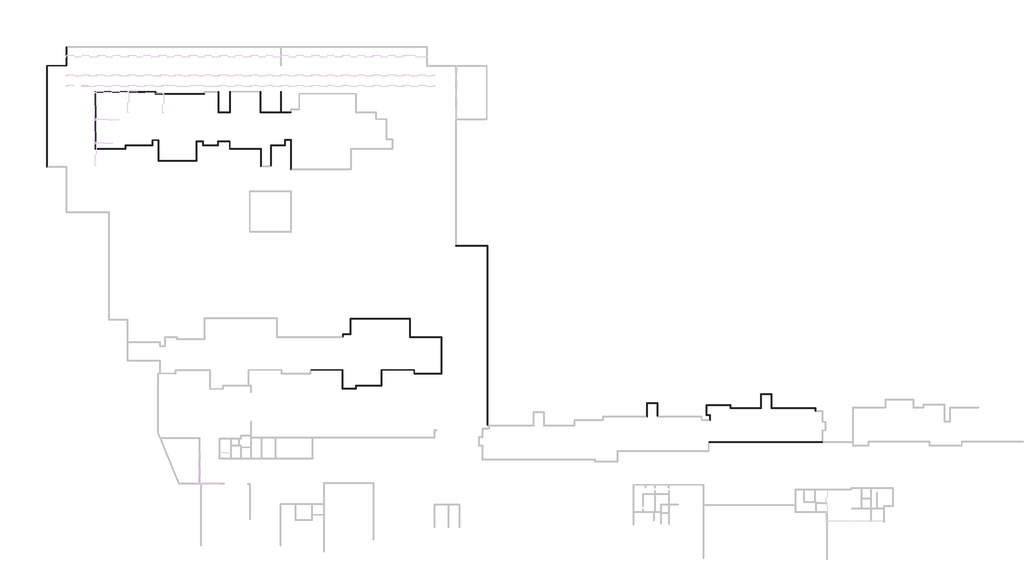
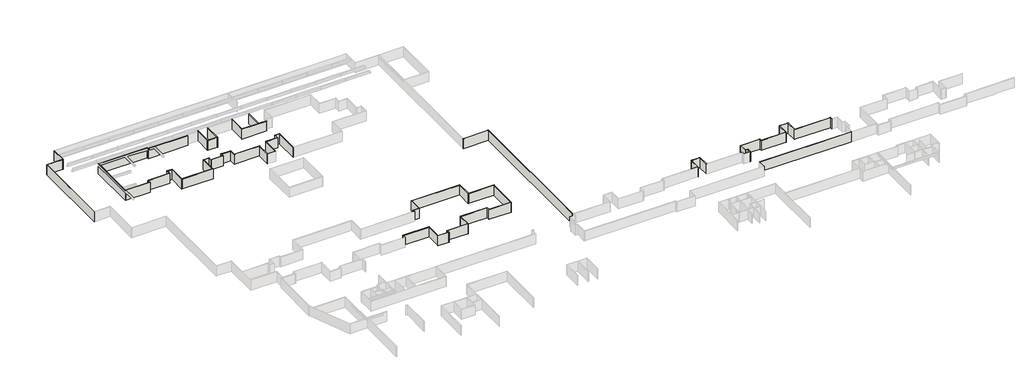
# One storey, part 5 of 8: 67 walls.
"""IFC4 building model written with IfcOpenShell, lengths in millimetres."""

from ifc_helpers import new_model, si_unit, origin, origin_with_axes, place, context, project, spatial, polyline, outline, extrude, faceted_brep, element, save

model = new_model("IFC4")

# Units and contexts
model_context = context("Model", 3, world=origin())
ifc_project = project(units=[si_unit("LENGTHUNIT", "METRE", prefix="MILLI")], contexts=[model_context])

# Site, building, storey
site = spatial("IfcSite", under=ifc_project)
building = spatial("IfcBuilding", under=site)
storey = spatial("IfcBuildingStorey", under=building, Name="户型图", Elevation=0.0)

# Walls
placement = place(None, origin())
element("IfcWall", 1, ObjectType="所有墙体", at=placement, inside=storey, context=model_context, shape_type="Brep", body=[
    faceted_brep([(57050.338145, 153057.0451916, 0.0), (57050.338145, 126907.0451941, 0.0), (57050.338145, 126907.0451941, 3300.0), (57050.338145, 153057.0451916, 3300.0), (57170.338145, 153057.0451916, 0.0), (57170.338145, 153057.0451916, 3300.0), (57170.338145, 127027.0451941, 3300.0), (57170.338145, 126907.0451941, 3300.0), (57170.338145, 126907.0451941, 0.0), (57170.338145, 127027.0451941, 0.0)], [[[0, 1, 2, 3]], [[4, 5, 6, 7, 8, 9]], [[1, 0, 4, 9, 8]], [[3, 2, 7, 6, 5]], [[2, 1, 8, 7]], [[0, 3, 5, 4]]]),
])
element("IfcWall", 2, ObjectType="所有墙体", at=placement, inside=storey, context=model_context, shape_type="Brep", body=[
    faceted_brep([(255784.4931741, 63876.5127734, 0.0), (255784.4931741, 64676.5110317, 0.0), (255784.4931741, 64676.5110317, 3300.0), (255784.4931741, 63876.5127734, 3300.0), (255664.4931741, 63876.5127734, 0.0), (255664.4931741, 63876.5127734, 3300.0), (255664.4931741, 64556.5110317, 3300.0), (255664.4931741, 64676.5110317, 3300.0), (255664.4931741, 64676.5110317, 0.0), (255664.4931741, 64556.5110317, 0.0)], [[[0, 1, 2, 3]], [[4, 5, 6, 7, 8, 9]], [[1, 0, 4, 9, 8]], [[3, 2, 7, 6, 5]], [[0, 3, 5, 4]], [[2, 1, 8, 7]]]),
])
element("IfcWall", 3, ObjectType="所有墙体", at=placement, inside=storey, context=model_context, shape_type="Brep", body=[
    faceted_brep([(255664.4931741, 64676.5110317, 0.0), (244359.4928017, 64676.5110317, 0.0), (244239.4928017, 64676.5110317, 0.0), (244239.4928017, 64676.5110317, 3300.0), (244359.4928017, 64676.5110317, 3300.0), (255664.4931741, 64676.5110317, 3300.0), (255664.4931741, 64556.5110317, 0.0), (255664.4931741, 64556.5110317, 3300.0), (244239.4928017, 64556.5110317, 3300.0), (244239.4928017, 64556.5110317, 0.0)], [[[0, 1, 2, 3, 4, 5]], [[6, 7, 8, 9]], [[2, 1, 0, 6, 9]], [[5, 4, 3, 8, 7]], [[0, 5, 7, 6]], [[3, 2, 9, 8]]]),
])
element("IfcWall", 4, ObjectType="所有墙体", at=placement, inside=storey, context=model_context, shape_type="Brep", body=[
    faceted_brep([(244359.4928017, 64676.5110317, 0.0), (244359.4928017, 68251.5115193, 0.0), (244359.4928017, 68251.5115193, 3300.0), (244359.4928017, 64676.5110317, 3300.0), (244239.4928017, 64676.5110317, 0.0), (244239.4928017, 64676.5110317, 3300.0), (244239.4928017, 68131.5115193, 3300.0), (244239.4928017, 68251.5115193, 3300.0), (244239.4928017, 68251.5115193, 0.0), (244239.4928017, 68131.5115193, 0.0)], [[[0, 1, 2, 3]], [[4, 5, 6, 7, 8, 9]], [[1, 0, 4, 9, 8]], [[3, 2, 7, 6, 5]], [[0, 3, 5, 4]], [[2, 1, 8, 7]]]),
])
element("IfcWall", 5, ObjectType="所有墙体", at=placement, inside=storey, context=model_context, shape_type="Brep", body=[
    faceted_brep([(244239.4928017, 68251.5115193, 0.0), (241539.4892961, 68251.5115193, 0.0), (241539.4892961, 68251.5115193, 3300.0), (244239.4928017, 68251.5115193, 3300.0), (244239.4928017, 68131.5115193, 0.0), (244239.4928017, 68131.5115193, 3300.0), (241659.4892961, 68131.5115193, 3300.0), (241539.4892961, 68131.5115193, 3300.0), (241539.4892961, 68131.5115193, 0.0), (241659.4892961, 68131.5115193, 0.0)], [[[0, 1, 2, 3]], [[4, 5, 6, 7, 8, 9]], [[1, 0, 4, 9, 8]], [[3, 2, 7, 6, 5]], [[0, 3, 5, 4]], [[2, 1, 8, 7]]]),
])
element("IfcWall", 6, ObjectType="所有墙体", at=placement, inside=storey, context=model_context, shape_type="Brep", body=[
    faceted_brep([(241539.4892961, 68131.5115193, 0.0), (241539.4892961, 64676.5110317, 0.0), (241539.4892961, 64556.5110317, 0.0), (241539.4892961, 64556.5110317, 3300.0), (241539.4892961, 64676.5110317, 3300.0), (241539.4892961, 68131.5115193, 3300.0), (241659.4892961, 68131.5115193, 0.0), (241659.4892961, 68131.5115193, 3300.0), (241659.4892961, 64556.5110317, 3300.0), (241659.4892961, 64556.5110317, 0.0)], [[[0, 1, 2, 3, 4, 5]], [[6, 7, 8, 9]], [[2, 1, 0, 6, 9]], [[5, 4, 3, 8, 7]], [[0, 5, 7, 6]], [[3, 2, 9, 8]]]),
])
element("IfcWall", 7, ObjectType="所有墙体", at=placement, inside=storey, context=model_context, shape_type="Brep", body=[
    faceted_brep([(241539.4892961, 64676.5110317, 0.0), (233784.2041334, 64676.5110317, 0.0), (233664.2041334, 64676.5110317, 0.0), (233664.2041334, 64676.5110317, 3300.0), (233784.2041334, 64676.5110317, 3300.0), (241539.4892961, 64676.5110317, 3300.0), (241539.4892961, 64556.5110317, 0.0), (241539.4892961, 64556.5110317, 3300.0), (233664.2041334, 64556.5110317, 3300.0), (233664.2041334, 64556.5110317, 0.0)], [[[0, 1, 2, 3, 4, 5]], [[6, 7, 8, 9]], [[2, 1, 0, 6, 9]], [[5, 4, 3, 8, 7]], [[0, 5, 7, 6]], [[3, 2, 9, 8]]]),
])
element("IfcWall", 8, ObjectType="所有墙体", at=placement, inside=storey, context=model_context, shape_type="Brep", body=[
    faceted_brep([(233784.2041334, 64676.5110317, 0.0), (233784.2041334, 65376.5510572, 0.0), (233784.2041334, 65376.5510572, 3300.0), (233784.2041334, 64676.5110317, 3300.0), (233664.2041334, 64676.5110317, 0.0), (233664.2041334, 64676.5110317, 3300.0), (233664.2041334, 65256.5510572, 3300.0), (233664.2041334, 65376.5510572, 3300.0), (233664.2041334, 65376.5510572, 0.0), (233664.2041334, 65256.5510572, 0.0)], [[[0, 1, 2, 3]], [[4, 5, 6, 7, 8, 9]], [[1, 0, 4, 9, 8]], [[3, 2, 7, 6, 5]], [[0, 3, 5, 4]], [[2, 1, 8, 7]]]),
])
element("IfcWall", 9, ObjectType="所有墙体", at=placement, inside=storey, context=model_context, shape_type="Brep", body=[
    faceted_brep([(233664.2041334, 65376.5510572, 0.0), (227494.4759798, 65376.5510572, 0.0), (227494.4759798, 65376.5510572, 3300.0), (233664.2041334, 65376.5510572, 3300.0), (233664.2041334, 65256.5510572, 0.0), (233664.2041334, 65256.5510572, 3300.0), (227614.4759798, 65256.5510572, 3300.0), (227494.4759798, 65256.5510572, 3300.0), (227494.4759798, 65256.5510572, 0.0), (227614.4759798, 65256.5510572, 0.0)], [[[0, 1, 2, 3]], [[4, 5, 6, 7, 8, 9]], [[1, 0, 4, 9, 8]], [[3, 2, 7, 6, 5]], [[0, 3, 5, 4]], [[2, 1, 8, 7]]]),
])
element("IfcWall", 10, ObjectType="所有墙体", at=placement, inside=storey, context=model_context, shape_type="Brep", body=[
    faceted_brep([(227494.4759798, 65256.5510572, 0.0), (227494.4759798, 62756.5107166, 0.0), (227494.4759798, 62756.5107166, 3300.0), (227494.4759798, 65256.5510572, 3300.0), (227614.4759798, 65256.5510572, 0.0), (227614.4759798, 65256.5510572, 3300.0), (227614.4759798, 62876.5107166, 3300.0), (227614.4759798, 62756.5107166, 3300.0), (227614.4759798, 62756.5107166, 0.0), (227614.4759798, 62876.5107166, 0.0)], [[[0, 1, 2, 3]], [[4, 5, 6, 7, 8, 9]], [[1, 0, 4, 9, 8]], [[3, 2, 7, 6, 5]], [[0, 3, 5, 4]], [[2, 1, 8, 7]]]),
])
element("IfcWall", 11, ObjectType="所有墙体", at=placement, inside=storey, context=model_context, shape_type="Brep", body=[
    faceted_brep([(227614.4759798, 62756.5107166, 0.0), (228364.4881621, 62756.5107166, 0.0), (228484.4881621, 62756.5107166, 0.0), (228484.4881621, 62756.5107166, 3300.0), (228364.4881621, 62756.5107166, 3300.0), (227614.4759798, 62756.5107166, 3300.0), (227614.4759798, 62876.5107166, 0.0), (227614.4759798, 62876.5107166, 3300.0), (228484.4881621, 62876.5107166, 3300.0), (228484.4881621, 62876.5107166, 0.0)], [[[0, 1, 2, 3, 4, 5]], [[6, 7, 8, 9]], [[2, 1, 0, 6, 9]], [[5, 4, 3, 8, 7]], [[0, 5, 7, 6]], [[3, 2, 9, 8]]]),
])
element("IfcWall", 12, ObjectType="所有墙体", at=placement, inside=storey, context=model_context, shape_type="Brep", body=[
    faceted_brep([(228364.4881621, 62756.5107166, 0.0), (228364.4881621, 61576.5107166, 0.0), (228364.4881621, 61456.5107166, 0.0), (228364.4881621, 61456.5107166, 3300.0), (228364.4881621, 61576.5107166, 3300.0), (228364.4881621, 62756.5107166, 3300.0), (228484.4881621, 62756.5107166, 0.0), (228484.4881621, 62756.5107166, 3300.0), (228484.4881621, 61456.5107166, 3300.0), (228484.4881621, 61456.5107166, 0.0)], [[[0, 1, 2, 3, 4, 5]], [[6, 7, 8, 9]], [[2, 1, 0, 6, 9]], [[5, 4, 3, 8, 7]], [[0, 5, 7, 6]], [[3, 2, 9, 8]]]),
])
element("IfcWall", 13, ObjectType="所有墙体", at=placement, inside=storey, context=model_context, shape_type="Brep", body=[
    faceted_brep([(214984.4914101, 62376.635741, 0.0), (214984.4914101, 65951.6356657, 0.0), (214984.4914101, 65951.6356657, 3300.0), (214984.4914101, 62376.635741, 3300.0), (214864.4914101, 62376.635741, 0.0), (214864.4914101, 62376.635741, 3300.0), (214864.4914101, 65831.6356657, 3300.0), (214864.4914101, 65951.6356657, 3300.0), (214864.4914101, 65951.6356657, 0.0), (214864.4914101, 65831.6356657, 0.0)], [[[0, 1, 2, 3]], [[4, 5, 6, 7, 8, 9]], [[1, 0, 4, 9, 8]], [[3, 2, 7, 6, 5]], [[0, 3, 5, 4]], [[2, 1, 8, 7]]]),
])
element("IfcWall", 14, ObjectType="所有墙体", at=placement, inside=storey, context=model_context, shape_type="Brep", body=[
    faceted_brep([(214864.4914101, 65951.6356657, 0.0), (212164.4916662, 65951.6356657, 0.0), (212164.4916662, 65951.6356657, 3300.0), (214864.4914101, 65951.6356657, 3300.0), (214864.4914101, 65831.6356657, 0.0), (214864.4914101, 65831.6356657, 3300.0), (212284.4916662, 65831.6356657, 3300.0), (212164.4916662, 65831.6356657, 3300.0), (212164.4916662, 65831.6356657, 0.0), (212284.4916662, 65831.6356657, 0.0)], [[[0, 1, 2, 3]], [[4, 5, 6, 7, 8, 9]], [[1, 0, 4, 9, 8]], [[3, 2, 7, 6, 5]], [[0, 3, 5, 4]], [[2, 1, 8, 7]]]),
])
element("IfcWall", 15, ObjectType="所有墙体", at=placement, inside=storey, context=model_context, shape_type="Brep", body=[
    faceted_brep([(212164.4916662, 65831.6356657, 0.0), (212164.4916662, 62376.635741, 0.0), (212164.4916662, 62256.635741, 0.0), (212164.4916662, 62256.635741, 3300.0), (212164.4916662, 62376.635741, 3300.0), (212164.4916662, 65831.6356657, 3300.0), (212284.4916662, 65831.6356657, 0.0), (212284.4916662, 65831.6356657, 3300.0), (212284.4916662, 62256.635741, 3300.0), (212284.4916662, 62256.635741, 0.0)], [[[0, 1, 2, 3, 4, 5]], [[6, 7, 8, 9]], [[2, 1, 0, 6, 9]], [[5, 4, 3, 8, 7]], [[0, 5, 7, 6]], [[3, 2, 9, 8]]]),
])
element("IfcWall", 16, ObjectType="所有墙体", at=placement, inside=storey, context=model_context, shape_type="Brep", body=[
    faceted_brep([(171033.8238906, 60076.635667, 0.0), (171033.8238906, 106576.635667, 0.0), (171033.8238906, 106576.635667, 3300.0), (171033.8238906, 60076.635667, 3300.0), (170913.8238906, 60076.635667, 0.0), (170913.8238906, 60076.635667, 3300.0), (170913.8238906, 106456.635667, 3300.0), (170913.8238906, 106576.635667, 3300.0), (170913.8238906, 106576.635667, 0.0), (170913.8238906, 106456.635667, 0.0)], [[[0, 1, 2, 3]], [[4, 5, 6, 7, 8, 9]], [[1, 0, 4, 9, 8]], [[3, 2, 7, 6, 5]], [[0, 3, 5, 4]], [[2, 1, 8, 7]]]),
])
element("IfcWall", 17, ObjectType="所有墙体", at=placement, inside=storey, context=model_context, shape_type="Brep", body=[
    faceted_brep([(170913.8238906, 106576.635667, 0.0), (162933.8477327, 106576.635667, 0.0), (162813.8477327, 106576.635667, 0.0), (162813.8477327, 106576.635667, 3300.0), (162933.8477327, 106576.635667, 3300.0), (170913.8238906, 106576.635667, 3300.0), (170913.8238906, 106456.635667, 0.0), (170913.8238906, 106456.635667, 3300.0), (162813.8477327, 106456.635667, 3300.0), (162813.8477327, 106456.635667, 0.0)], [[[0, 1, 2, 3, 4, 5]], [[6, 7, 8, 9]], [[2, 1, 0, 6, 9]], [[5, 4, 3, 8, 7]], [[0, 5, 7, 6]], [[3, 2, 9, 8]]]),
])
element("IfcWall", 18, ObjectType="所有墙体", at=placement, inside=storey, context=model_context, shape_type="Brep", body=[
    faceted_brep([(62138.8476291, 157956.8472847, 0.0), (62138.8476291, 153177.0451916, 0.0), (62138.8476291, 153057.0451916, 0.0), (62138.8476291, 153057.0451916, 3300.0), (62138.8476291, 153177.0451916, 3300.0), (62138.8476291, 157956.8472847, 3300.0), (62258.8476291, 157956.8472847, 0.0), (62258.8476291, 157956.8472847, 3300.0), (62258.8476291, 153057.0451916, 3300.0), (62258.8476291, 153057.0451916, 0.0)], [[[0, 1, 2, 3, 4, 5]], [[6, 7, 8, 9]], [[2, 1, 0, 6, 9]], [[5, 4, 3, 8, 7]], [[0, 5, 7, 6]], [[3, 2, 9, 8]]]),
])
element("IfcWall", 19, ObjectType="所有墙体", at=placement, inside=storey, context=model_context, shape_type="SweptSolid", body=[
    extrude(outline(polyline([(57050.338145, 153177.0451916), (62138.8476291, 153177.0451916), (62138.8476291, 153057.0451916), (57050.338145, 153057.0451916), (57050.338145, 153177.0451916)])), origin_with_axes(), (0.0, 0.0, 1.0), 3300.0),
])
element("IfcWall", 20, ObjectType="所有墙体", at=placement, inside=storey, context=model_context, shape_type="Brep", body=[
    faceted_brep([(69623.6976621, 146403.9951293, 0.0), (69623.6976621, 131534.2446453, 0.0), (69623.6976621, 131534.2446453, 3300.0), (69623.6976621, 146403.9951293, 3300.0), (69743.6976621, 146403.9951293, 0.0), (69743.6976621, 146403.9951293, 3300.0), (69743.6976621, 146283.9951293, 3300.0), (69743.6976621, 131654.2446453, 3300.0), (69743.6976621, 131534.2446453, 3300.0), (69743.6976621, 131534.2446453, 0.0), (69743.6976621, 131654.2446453, 0.0), (69743.6976621, 146283.9951293, 0.0)], [[[0, 1, 2, 3]], [[4, 5, 6, 7, 8, 9, 10, 11]], [[1, 0, 4, 11, 10, 9]], [[3, 2, 8, 7, 6, 5]], [[2, 1, 9, 8]], [[0, 3, 5, 4]]]),
])
element("IfcWall", 21, ObjectType="所有墙体", at=placement, inside=storey, context=model_context, shape_type="Brep", body=[
    faceted_brep([(69743.6976621, 131534.2446453, 0.0), (77542.6046485, 131534.2446453, 0.0), (77542.6046485, 131534.2446453, 3300.0), (69743.6976621, 131534.2446453, 3300.0), (69743.6976621, 131654.2446453, 0.0), (69743.6976621, 131654.2446453, 3300.0), (77422.6046485, 131654.2446453, 3300.0), (77542.6046485, 131654.2446453, 3300.0), (77542.6046485, 131654.2446453, 0.0), (77422.6046485, 131654.2446453, 0.0)], [[[0, 1, 2, 3]], [[4, 5, 6, 7, 8, 9]], [[1, 0, 4, 9, 8]], [[3, 2, 7, 6, 5]], [[0, 3, 5, 4]], [[2, 1, 8, 7]]]),
])
element("IfcWall", 22, ObjectType="所有墙体", at=placement, inside=storey, context=model_context, shape_type="Brep", body=[
    faceted_brep([(77542.6046485, 131654.2446453, 0.0), (77542.6046485, 132483.9951277, 0.0), (77542.6046485, 132603.9951277, 0.0), (77542.6046485, 132603.9951277, 3300.0), (77542.6046485, 132483.9951277, 3300.0), (77542.6046485, 131654.2446453, 3300.0), (77422.6046485, 131654.2446453, 0.0), (77422.6046485, 131654.2446453, 3300.0), (77422.6046485, 132603.9951277, 3300.0), (77422.6046485, 132603.9951277, 0.0)], [[[0, 1, 2, 3, 4, 5]], [[6, 7, 8, 9]], [[2, 1, 0, 6, 9]], [[5, 4, 3, 8, 7]], [[0, 5, 7, 6]], [[3, 2, 9, 8]]]),
])
element("IfcWall", 23, ObjectType="所有墙体", at=placement, inside=storey, context=model_context, shape_type="Brep", body=[
    faceted_brep([(77542.6046485, 132483.9951277, 0.0), (84442.604647, 132483.9951277, 0.0), (84442.604647, 132483.9951277, 3300.0), (77542.6046485, 132483.9951277, 3300.0), (77542.6046485, 132603.9951277, 0.0), (77542.6046485, 132603.9951277, 3300.0), (84322.604647, 132603.9951277, 3300.0), (84442.604647, 132603.9951277, 3300.0), (84442.604647, 132603.9951277, 0.0), (84322.604647, 132603.9951277, 0.0)], [[[0, 1, 2, 3]], [[4, 5, 6, 7, 8, 9]], [[1, 0, 4, 9, 8]], [[3, 2, 7, 6, 5]], [[0, 3, 5, 4]], [[2, 1, 8, 7]]]),
])
element("IfcWall", 24, ObjectType="所有墙体", at=placement, inside=storey, context=model_context, shape_type="Brep", body=[
    faceted_brep([(84442.604647, 132603.9951277, 0.0), (84442.604647, 133809.2583754, 0.0), (84442.604647, 133929.2583754, 0.0), (84442.604647, 133929.2583754, 3300.0), (84442.604647, 133809.2583754, 3300.0), (84442.604647, 132603.9951277, 3300.0), (84322.604647, 132603.9951277, 0.0), (84322.604647, 132603.9951277, 3300.0), (84322.604647, 133929.2583754, 3300.0), (84322.604647, 133929.2583754, 0.0)], [[[0, 1, 2, 3, 4, 5]], [[6, 7, 8, 9]], [[2, 1, 0, 6, 9]], [[5, 4, 3, 8, 7]], [[0, 5, 7, 6]], [[3, 2, 9, 8]]]),
])
element("IfcWall", 25, ObjectType="所有墙体", at=placement, inside=storey, context=model_context, shape_type="Brep", body=[
    faceted_brep([(84442.604647, 133809.2583754, 0.0), (85872.8500926, 133809.2583754, 0.0), (85992.8500926, 133809.2583754, 0.0), (85992.8500926, 133809.2583754, 3300.0), (85872.8500926, 133809.2583754, 3300.0), (84442.604647, 133809.2583754, 3300.0), (84442.604647, 133929.2583754, 0.0), (84442.604647, 133929.2583754, 3300.0), (85992.8500926, 133929.2583754, 3300.0), (85992.8500926, 133929.2583754, 0.0)], [[[0, 1, 2, 3, 4, 5]], [[6, 7, 8, 9]], [[2, 1, 0, 6, 9]], [[5, 4, 3, 8, 7]], [[0, 5, 7, 6]], [[3, 2, 9, 8]]]),
])
element("IfcWall", 26, ObjectType="所有墙体", at=placement, inside=storey, context=model_context, shape_type="Brep", body=[
    faceted_brep([(85872.8500926, 133809.2583754, 0.0), (85872.8500926, 128433.7456138, 0.0), (85872.8500926, 128433.7456138, 3300.0), (85872.8500926, 133809.2583754, 3300.0), (85992.8500926, 133809.2583754, 0.0), (85992.8500926, 133809.2583754, 3300.0), (85992.8500926, 128553.7456138, 3300.0), (85992.8500926, 128433.7456138, 3300.0), (85992.8500926, 128433.7456138, 0.0), (85992.8500926, 128553.7456138, 0.0)], [[[0, 1, 2, 3]], [[4, 5, 6, 7, 8, 9]], [[1, 0, 4, 9, 8]], [[3, 2, 7, 6, 5]], [[0, 3, 5, 4]], [[2, 1, 8, 7]]]),
])
element("IfcWall", 27, ObjectType="所有墙体", at=placement, inside=storey, context=model_context, shape_type="Brep", body=[
    faceted_brep([(85992.8500926, 128433.7456138, 0.0), (95842.6046456, 128433.7456138, 0.0), (95842.6046456, 128433.7456138, 3300.0), (85992.8500926, 128433.7456138, 3300.0), (85992.8500926, 128553.7456138, 0.0), (85992.8500926, 128553.7456138, 3300.0), (95722.6046456, 128553.7456138, 3300.0), (95842.6046456, 128553.7456138, 3300.0), (95842.6046456, 128553.7456138, 0.0), (95722.6046456, 128553.7456138, 0.0)], [[[0, 1, 2, 3]], [[4, 5, 6, 7, 8, 9]], [[1, 0, 4, 9, 8]], [[3, 2, 7, 6, 5]], [[0, 3, 5, 4]], [[2, 1, 8, 7]]]),
])
element("IfcWall", 28, ObjectType="所有墙体", at=placement, inside=storey, context=model_context, shape_type="Brep", body=[
    faceted_brep([(95842.6046456, 128553.7456138, 0.0), (95842.6046456, 133459.9748435, 0.0), (95842.6046456, 133579.9748435, 0.0), (95842.6046456, 133579.9748435, 3300.0), (95842.6046456, 133459.9748435, 3300.0), (95842.6046456, 128553.7456138, 3300.0), (95722.6046456, 128553.7456138, 0.0), (95722.6046456, 128553.7456138, 3300.0), (95722.6046456, 133579.9748435, 3300.0), (95722.6046456, 133579.9748435, 0.0)], [[[0, 1, 2, 3, 4, 5]], [[6, 7, 8, 9]], [[2, 1, 0, 6, 9]], [[5, 4, 3, 8, 7]], [[0, 5, 7, 6]], [[3, 2, 9, 8]]]),
])
element("IfcWall", 29, ObjectType="所有墙体", at=placement, inside=storey, context=model_context, shape_type="Brep", body=[
    faceted_brep([(95842.6046456, 133459.9748435, 0.0), (97422.6046504, 133459.9748435, 0.0), (97542.6046504, 133459.9748435, 0.0), (97542.6046504, 133459.9748435, 3300.0), (97422.6046504, 133459.9748435, 3300.0), (95842.6046456, 133459.9748435, 3300.0), (95842.6046456, 133579.9748435, 0.0), (95842.6046456, 133579.9748435, 3300.0), (97542.6046504, 133579.9748435, 3300.0), (97542.6046504, 133579.9748435, 0.0)], [[[0, 1, 2, 3, 4, 5]], [[6, 7, 8, 9]], [[2, 1, 0, 6, 9]], [[5, 4, 3, 8, 7]], [[0, 5, 7, 6]], [[3, 2, 9, 8]]]),
])
element("IfcWall", 30, ObjectType="所有墙体", at=placement, inside=storey, context=model_context, shape_type="Brep", body=[
    faceted_brep([(97422.6046504, 133459.9748435, 0.0), (97422.6046504, 132483.9951277, 0.0), (97422.6046504, 132483.9951277, 3300.0), (97422.6046504, 133459.9748435, 3300.0), (97542.6046504, 133459.9748435, 0.0), (97542.6046504, 133459.9748435, 3300.0), (97542.6046504, 132603.9951277, 3300.0), (97542.6046504, 132483.9951277, 3300.0), (97542.6046504, 132483.9951277, 0.0), (97542.6046504, 132603.9951277, 0.0)], [[[0, 1, 2, 3]], [[4, 5, 6, 7, 8, 9]], [[1, 0, 4, 9, 8]], [[3, 2, 7, 6, 5]], [[0, 3, 5, 4]], [[2, 1, 8, 7]]]),
])
element("IfcWall", 31, ObjectType="所有墙体", at=placement, inside=storey, context=model_context, shape_type="Brep", body=[
    faceted_brep([(97542.6046504, 132483.9951277, 0.0), (101442.5262147, 132483.9951277, 0.0), (101442.5262147, 132483.9951277, 3300.0), (97542.6046504, 132483.9951277, 3300.0), (97542.6046504, 132603.9951277, 0.0), (97542.6046504, 132603.9951277, 3300.0), (101322.5262147, 132603.9951277, 3300.0), (101442.5262147, 132603.9951277, 3300.0), (101442.5262147, 132603.9951277, 0.0), (101322.5262147, 132603.9951277, 0.0)], [[[0, 1, 2, 3]], [[4, 5, 6, 7, 8, 9]], [[1, 0, 4, 9, 8]], [[3, 2, 7, 6, 5]], [[0, 3, 5, 4]], [[2, 1, 8, 7]]]),
])
element("IfcWall", 32, ObjectType="所有墙体", at=placement, inside=storey, context=model_context, shape_type="Brep", body=[
    faceted_brep([(101442.5262147, 132603.9951277, 0.0), (101442.5262147, 133459.9748435, 0.0), (101442.5262147, 133579.9748435, 0.0), (101442.5262147, 133579.9748435, 3300.0), (101442.5262147, 133459.9748435, 3300.0), (101442.5262147, 132603.9951277, 3300.0), (101322.5262147, 132603.9951277, 0.0), (101322.5262147, 132603.9951277, 3300.0), (101322.5262147, 133579.9748435, 3300.0), (101322.5262147, 133579.9748435, 0.0)], [[[0, 1, 2, 3, 4, 5]], [[6, 7, 8, 9]], [[2, 1, 0, 6, 9]], [[5, 4, 3, 8, 7]], [[0, 5, 7, 6]], [[3, 2, 9, 8]]]),
])
element("IfcWall", 33, ObjectType="所有墙体", at=placement, inside=storey, context=model_context, shape_type="Brep", body=[
    faceted_brep([(101442.5262147, 133459.9748435, 0.0), (104322.6046472, 133459.9748435, 0.0), (104442.6046472, 133459.9748435, 0.0), (104442.6046472, 133459.9748435, 3300.0), (104322.6046472, 133459.9748435, 3300.0), (101442.5262147, 133459.9748435, 3300.0), (101442.5262147, 133579.9748435, 0.0), (101442.5262147, 133579.9748435, 3300.0), (104442.6046472, 133579.9748435, 3300.0), (104442.6046472, 133579.9748435, 0.0)], [[[0, 1, 2, 3, 4, 5]], [[6, 7, 8, 9]], [[2, 1, 0, 6, 9]], [[5, 4, 3, 8, 7]], [[0, 5, 7, 6]], [[3, 2, 9, 8]]]),
])
element("IfcWall", 34, ObjectType="所有墙体", at=placement, inside=storey, context=model_context, shape_type="Brep", body=[
    faceted_brep([(104322.6046472, 133459.9748435, 0.0), (104322.6046472, 131533.7456111, 0.0), (104322.6046472, 131533.7456111, 3300.0), (104322.6046472, 133459.9748435, 3300.0), (104442.6046472, 133459.9748435, 0.0), (104442.6046472, 133459.9748435, 3300.0), (104442.6046472, 131653.7456111, 3300.0), (104442.6046472, 131533.7456111, 3300.0), (104442.6046472, 131533.7456111, 0.0), (104442.6046472, 131653.7456111, 0.0)], [[[0, 1, 2, 3]], [[4, 5, 6, 7, 8, 9]], [[1, 0, 4, 9, 8]], [[3, 2, 7, 6, 5]], [[0, 3, 5, 4]], [[2, 1, 8, 7]]]),
])
element("IfcWall", 35, ObjectType="所有墙体", at=placement, inside=storey, context=model_context, shape_type="Brep", body=[
    faceted_brep([(104442.6046472, 131533.7456111, 0.0), (112388.8239737, 131533.7456111, 0.0), (112508.8239737, 131533.7456111, 0.0), (112508.8239737, 131533.7456111, 3300.0), (112388.8239737, 131533.7456111, 3300.0), (104442.6046472, 131533.7456111, 3300.0), (104442.6046472, 131653.7456111, 0.0), (104442.6046472, 131653.7456111, 3300.0), (112508.8239737, 131653.7456111, 3300.0), (112508.8239737, 131653.7456111, 0.0)], [[[0, 1, 2, 3, 4, 5]], [[6, 7, 8, 9]], [[2, 1, 0, 6, 9]], [[5, 4, 3, 8, 7]], [[0, 5, 7, 6]], [[3, 2, 9, 8]]]),
])
element("IfcWall", 36, ObjectType="所有墙体", at=placement, inside=storey, context=model_context, shape_type="Brep", body=[
    faceted_brep([(112388.8239737, 131533.7456111, 0.0), (112388.8239737, 127056.6496336, 0.0), (112388.8239737, 127056.6496336, 3300.0), (112388.8239737, 131533.7456111, 3300.0), (112508.8239737, 131533.7456111, 0.0), (112508.8239737, 131533.7456111, 3300.0), (112508.8239737, 127176.6496336, 3300.0), (112508.8239737, 127056.6496336, 3300.0), (112508.8239737, 127056.6496336, 0.0), (112508.8239737, 127176.6496336, 0.0)], [[[0, 1, 2, 3]], [[4, 5, 6, 7, 8, 9]], [[1, 0, 4, 9, 8]], [[3, 2, 7, 6, 5]], [[0, 3, 5, 4]], [[2, 1, 8, 7]]]),
])
element("IfcWall", 37, ObjectType="所有墙体", at=placement, inside=storey, context=model_context, shape_type="Brep", body=[
    faceted_brep([(115083.8238911, 127176.6496336, 0.0), (115083.8238911, 132483.9951277, 0.0), (115083.8238911, 132603.9951277, 0.0), (115083.8238911, 132603.9951277, 3300.0), (115083.8238911, 132483.9951277, 3300.0), (115083.8238911, 127176.6496336, 3300.0), (114963.8238911, 127176.6496336, 0.0), (114963.8238911, 127176.6496336, 3300.0), (114963.8238911, 132603.9951277, 3300.0), (114963.8238911, 132603.9951277, 0.0)], [[[0, 1, 2, 3, 4, 5]], [[6, 7, 8, 9]], [[2, 1, 0, 6, 9]], [[5, 4, 3, 8, 7]], [[0, 5, 7, 6]], [[3, 2, 9, 8]]]),
])
element("IfcWall", 38, ObjectType="所有墙体", at=placement, inside=storey, context=model_context, shape_type="Brep", body=[
    faceted_brep([(115083.8238911, 132483.9951277, 0.0), (118752.6046466, 132483.9951277, 0.0), (118752.6046466, 132483.9951277, 3300.0), (115083.8238911, 132483.9951277, 3300.0), (115083.8238911, 132603.9951277, 0.0), (115083.8238911, 132603.9951277, 3300.0), (118632.6046466, 132603.9951277, 3300.0), (118752.6046466, 132603.9951277, 3300.0), (118752.6046466, 132603.9951277, 0.0), (118632.6046466, 132603.9951277, 0.0)], [[[0, 1, 2, 3]], [[4, 5, 6, 7, 8, 9]], [[1, 0, 4, 9, 8]], [[3, 2, 7, 6, 5]], [[0, 3, 5, 4]], [[2, 1, 8, 7]]]),
])
element("IfcWall", 39, ObjectType="所有墙体", at=placement, inside=storey, context=model_context, shape_type="Brep", body=[
    faceted_brep([(118752.6046466, 132603.9951277, 0.0), (118752.6046466, 133884.2446429, 0.0), (118752.6046466, 134004.2446429, 0.0), (118752.6046466, 134004.2446429, 3300.0), (118752.6046466, 133884.2446429, 3300.0), (118752.6046466, 132603.9951277, 3300.0), (118632.6046466, 132603.9951277, 0.0), (118632.6046466, 132603.9951277, 3300.0), (118632.6046466, 134004.2446429, 3300.0), (118632.6046466, 134004.2446429, 0.0)], [[[0, 1, 2, 3, 4, 5]], [[6, 7, 8, 9]], [[2, 1, 0, 6, 9]], [[5, 4, 3, 8, 7]], [[0, 5, 7, 6]], [[3, 2, 9, 8]]]),
])
element("IfcWall", 40, ObjectType="所有墙体", at=placement, inside=storey, context=model_context, shape_type="Brep", body=[
    faceted_brep([(118752.6046466, 133884.2446429, 0.0), (120132.3761316, 133884.2446429, 0.0), (120252.3761316, 133884.2446429, 0.0), (120252.3761316, 133884.2446429, 3300.0), (120132.3761316, 133884.2446429, 3300.0), (118752.6046466, 133884.2446429, 3300.0), (118752.6046466, 134004.2446429, 0.0), (118752.6046466, 134004.2446429, 3300.0), (120252.3761316, 134004.2446429, 3300.0), (120252.3761316, 134004.2446429, 0.0)], [[[0, 1, 2, 3, 4, 5]], [[6, 7, 8, 9]], [[2, 1, 0, 6, 9]], [[5, 4, 3, 8, 7]], [[0, 5, 7, 6]], [[3, 2, 9, 8]]]),
])
element("IfcWall", 41, ObjectType="所有墙体", at=placement, inside=storey, context=model_context, shape_type="Brep", body=[
    faceted_brep([(120132.3761316, 133884.2446429, 0.0), (120132.3761316, 126236.2446076, 0.0), (120132.3761316, 126236.2446076, 3300.0), (120132.3761316, 133884.2446429, 3300.0), (120252.3761316, 133884.2446429, 0.0), (120252.3761316, 133884.2446429, 3300.0), (120252.3761316, 126356.2446076, 3300.0), (120252.3761316, 126236.2446076, 3300.0), (120252.3761316, 126236.2446076, 0.0), (120252.3761316, 126356.2446076, 0.0)], [[[0, 1, 2, 3]], [[4, 5, 6, 7, 8, 9]], [[1, 0, 4, 9, 8]], [[3, 2, 7, 6, 5]], [[0, 3, 5, 4]], [[2, 1, 8, 7]]]),
])
element("IfcWall", 42, ObjectType="所有墙体", at=placement, inside=storey, context=model_context, shape_type="Brep", body=[
    faceted_brep([(120182.8546857, 141104.2446487, 0.0), (117696.3185581, 141104.2446487, 0.0), (117576.3185581, 141104.2446487, 0.0), (112358.82396, 141104.2446487, 0.0), (112238.82396, 141104.2446487, 0.0), (112238.82396, 141104.2446487, 3300.0), (112358.82396, 141104.2446487, 3300.0), (117576.3185581, 141104.2446487, 3300.0), (117696.3185581, 141104.2446487, 3300.0), (120182.8546857, 141104.2446487, 3300.0), (120182.8546857, 140984.2446487, 0.0), (120182.8546857, 140984.2446487, 3300.0), (112238.82396, 140984.2446487, 3300.0), (112238.82396, 140984.2446487, 0.0)], [[[0, 1, 2, 3, 4, 5, 6, 7, 8, 9]], [[10, 11, 12, 13]], [[4, 3, 2, 1, 0, 10, 13]], [[9, 8, 7, 6, 5, 12, 11]], [[0, 9, 11, 10]], [[5, 4, 13, 12]]]),
])
element("IfcWall", 43, ObjectType="所有墙体", at=placement, inside=storey, context=model_context, shape_type="Brep", body=[
    faceted_brep([(112358.82396, 141104.2446487, 0.0), (112358.82396, 146454.2446479, 0.0), (112358.82396, 146454.2446479, 3300.0), (112358.82396, 141104.2446487, 3300.0), (112238.82396, 141104.2446487, 0.0), (112238.82396, 141104.2446487, 3300.0), (112238.82396, 146334.2446479, 3300.0), (112238.82396, 146454.2446479, 3300.0), (112238.82396, 146454.2446479, 0.0), (112238.82396, 146334.2446479, 0.0)], [[[0, 1, 2, 3]], [[4, 5, 6, 7, 8, 9]], [[1, 0, 4, 9, 8]], [[3, 2, 7, 6, 5]], [[0, 3, 5, 4]], [[2, 1, 8, 7]]]),
])
element("IfcWall", 44, ObjectType="所有墙体", at=placement, inside=storey, context=model_context, shape_type="Brep", body=[
    faceted_brep([(104388.8715153, 146334.2446479, 0.0), (104388.8715153, 141104.2446487, 0.0), (104388.8715153, 140984.2446487, 0.0), (104388.8715153, 140984.2446487, 3300.0), (104388.8715153, 141104.2446487, 3300.0), (104388.8715153, 146334.2446479, 3300.0), (104508.8715153, 146334.2446479, 0.0), (104508.8715153, 146334.2446479, 3300.0), (104508.8715153, 140984.2446487, 3300.0), (104508.8715153, 140984.2446487, 0.0)], [[[0, 1, 2, 3, 4, 5]], [[6, 7, 8, 9]], [[2, 1, 0, 6, 9]], [[5, 4, 3, 8, 7]], [[0, 5, 7, 6]], [[3, 2, 9, 8]]]),
])
element("IfcWall", 45, ObjectType="所有墙体", at=placement, inside=storey, context=model_context, shape_type="Brep", body=[
    faceted_brep([(104388.8715153, 141104.2446487, 0.0), (101492.8755148, 141104.2446487, 0.0), (101372.8755148, 141104.2446487, 0.0), (101372.8755148, 141104.2446487, 3300.0), (101492.8755148, 141104.2446487, 3300.0), (104388.8715153, 141104.2446487, 3300.0), (104388.8715153, 140984.2446487, 0.0), (104388.8715153, 140984.2446487, 3300.0), (101372.8755148, 140984.2446487, 3300.0), (101372.8755148, 140984.2446487, 0.0)], [[[0, 1, 2, 3, 4, 5]], [[6, 7, 8, 9]], [[2, 1, 0, 6, 9]], [[5, 4, 3, 8, 7]], [[0, 5, 7, 6]], [[3, 2, 9, 8]]]),
])
element("IfcWall", 46, ObjectType="所有墙体", at=placement, inside=storey, context=model_context, shape_type="Brep", body=[
    faceted_brep([(101492.8755148, 141104.2446487, 0.0), (101492.8755148, 146404.244647, 0.0), (101492.8755148, 146404.244647, 3300.0), (101492.8755148, 141104.2446487, 3300.0), (101372.8755148, 141104.2446487, 0.0), (101372.8755148, 141104.2446487, 3300.0), (101372.8755148, 146284.244647, 3300.0), (101372.8755148, 146404.244647, 3300.0), (101372.8755148, 146404.244647, 0.0), (101372.8755148, 146284.244647, 0.0)], [[[0, 1, 2, 3]], [[4, 5, 6, 7, 8, 9]], [[1, 0, 4, 9, 8]], [[3, 2, 7, 6, 5]], [[0, 3, 5, 4]], [[2, 1, 8, 7]]]),
])
element("IfcWall", 47, ObjectType="所有墙体", at=placement, inside=storey, context=model_context, shape_type="Brep", body=[
    faceted_brep([(97832.8755148, 145903.9951293, 0.0), (85242.7452463, 145903.9951293, 0.0), (85122.7452463, 145903.9951293, 0.0), (85122.7452463, 145903.9951293, 3300.0), (85242.7452463, 145903.9951293, 3300.0), (97832.8755148, 145903.9951293, 3300.0), (97832.8755148, 145783.9951293, 0.0), (97832.8755148, 145783.9951293, 3300.0), (85122.7452463, 145783.9951293, 3300.0), (85122.7452463, 145783.9951293, 0.0)], [[[0, 1, 2, 3, 4, 5]], [[6, 7, 8, 9]], [[2, 1, 0, 6, 9]], [[5, 4, 3, 8, 7]], [[0, 5, 7, 6]], [[3, 2, 9, 8]]]),
])
element("IfcWall", 48, ObjectType="所有墙体", at=placement, inside=storey, context=model_context, shape_type="Brep", body=[
    faceted_brep([(85242.7452463, 145903.9951293, 0.0), (85242.7452463, 146403.9951293, 0.0), (85242.7452463, 146403.9951293, 3300.0), (85242.7452463, 145903.9951293, 3300.0), (85122.7452463, 145903.9951293, 0.0), (85122.7452463, 145903.9951293, 3300.0), (85122.7452463, 146283.9951293, 3300.0), (85122.7452463, 146403.9951293, 3300.0), (85122.7452463, 146403.9951293, 0.0), (85122.7452463, 146283.9951293, 0.0)], [[[0, 1, 2, 3]], [[4, 5, 6, 7, 8, 9]], [[1, 0, 4, 9, 8]], [[3, 2, 7, 6, 5]], [[0, 3, 5, 4]], [[2, 1, 8, 7]]]),
])
element("IfcWall", 49, ObjectType="所有墙体", at=placement, inside=storey, context=model_context, shape_type="SweptSolid", body=[
    extrude(outline(polyline([(69743.6976621, 146403.9951293), (85122.7452463, 146403.9951293), (85122.7452463, 146283.9951293), (69743.6976621, 146283.9951293), (69743.6976621, 146403.9951293)])), origin_with_axes(), (0.0, 0.0, 1.0), 3300.0),
])
element("IfcWall", 50, ObjectType="所有墙体", at=placement, inside=storey, context=model_context, shape_type="Brep", body=[
    faceted_brep([(133740.1629656, 83008.343556, 0.0), (133740.1629656, 83589.6458208, 0.0), (133740.1629656, 83709.6458208, 0.0), (133740.1629656, 83709.6458208, 3300.0), (133740.1629656, 83589.6458208, 3300.0), (133740.1629656, 83008.343556, 3300.0), (133620.1629656, 83008.343556, 0.0), (133620.1629656, 83008.343556, 3300.0), (133620.1629656, 83709.6458208, 3300.0), (133620.1629656, 83709.6458208, 0.0)], [[[0, 1, 2, 3, 4, 5]], [[6, 7, 8, 9]], [[2, 1, 0, 6, 9]], [[5, 4, 3, 8, 7]], [[0, 5, 7, 6]], [[3, 2, 9, 8]]]),
])
element("IfcWall", 51, ObjectType="所有墙体", at=placement, inside=storey, context=model_context, shape_type="Brep", body=[
    faceted_brep([(133740.1629656, 83589.6458208, 0.0), (135649.986369, 83589.6458208, 0.0), (135649.986369, 83589.6458208, 3300.0), (133740.1629656, 83589.6458208, 3300.0), (133740.1629656, 83709.6458208, 0.0), (133740.1629656, 83709.6458208, 3300.0), (135529.986369, 83709.6458208, 3300.0), (135649.986369, 83709.6458208, 3300.0), (135649.986369, 83709.6458208, 0.0), (135529.986369, 83709.6458208, 0.0)], [[[0, 1, 2, 3]], [[4, 5, 6, 7, 8, 9]], [[1, 0, 4, 9, 8]], [[3, 2, 7, 6, 5]], [[0, 3, 5, 4]], [[2, 1, 8, 7]]]),
])
element("IfcWall", 52, ObjectType="所有墙体", at=placement, inside=storey, context=model_context, shape_type="Brep", body=[
    faceted_brep([(135649.986369, 83709.6458208, 0.0), (135649.986369, 87640.0782767, 0.0), (135649.986369, 87760.0782767, 0.0), (135649.986369, 87760.0782767, 3300.0), (135649.986369, 87640.0782767, 3300.0), (135649.986369, 83709.6458208, 3300.0), (135529.986369, 83709.6458208, 0.0), (135529.986369, 83709.6458208, 3300.0), (135529.986369, 87760.0782767, 3300.0), (135529.986369, 87760.0782767, 0.0)], [[[0, 1, 2, 3, 4, 5]], [[6, 7, 8, 9]], [[2, 1, 0, 6, 9]], [[5, 4, 3, 8, 7]], [[0, 5, 7, 6]], [[3, 2, 9, 8]]]),
])
element("IfcWall", 53, ObjectType="所有墙体", at=placement, inside=storey, context=model_context, shape_type="Brep", body=[
    faceted_brep([(135649.986369, 87640.0782767, 0.0), (150889.986369, 87640.0782767, 0.0), (151009.986369, 87640.0782767, 0.0), (151009.986369, 87640.0782767, 3300.0), (150889.986369, 87640.0782767, 3300.0), (135649.986369, 87640.0782767, 3300.0), (135649.986369, 87760.0782767, 0.0), (135649.986369, 87760.0782767, 3300.0), (151009.986369, 87760.0782767, 3300.0), (151009.986369, 87760.0782767, 0.0)], [[[0, 1, 2, 3, 4, 5]], [[6, 7, 8, 9]], [[2, 1, 0, 6, 9]], [[5, 4, 3, 8, 7]], [[0, 5, 7, 6]], [[3, 2, 9, 8]]]),
])
element("IfcWall", 54, ObjectType="所有墙体", at=placement, inside=storey, context=model_context, shape_type="Brep", body=[
    faceted_brep([(150889.986369, 87640.0782767, 0.0), (150889.986369, 82840.0782767, 0.0), (150889.986369, 82840.0782767, 3300.0), (150889.986369, 87640.0782767, 3300.0), (151009.986369, 87640.0782767, 0.0), (151009.986369, 87640.0782767, 3300.0), (151009.986369, 82960.0782767, 3300.0), (151009.986369, 82840.0782767, 3300.0), (151009.986369, 82840.0782767, 0.0), (151009.986369, 82960.0782767, 0.0)], [[[0, 1, 2, 3]], [[4, 5, 6, 7, 8, 9]], [[1, 0, 4, 9, 8]], [[3, 2, 7, 6, 5]], [[0, 3, 5, 4]], [[2, 1, 8, 7]]]),
])
element("IfcWall", 55, ObjectType="所有墙体", at=placement, inside=storey, context=model_context, shape_type="Brep", body=[
    faceted_brep([(151009.986369, 82840.0782767, 0.0), (159013.8473255, 82840.0782767, 0.0), (159133.8473255, 82840.0782767, 0.0), (159133.8473255, 82840.0782767, 3300.0), (159013.8473255, 82840.0782767, 3300.0), (151009.986369, 82840.0782767, 3300.0), (151009.986369, 82960.0782767, 0.0), (151009.986369, 82960.0782767, 3300.0), (159133.8473255, 82960.0782767, 3300.0), (159133.8473255, 82960.0782767, 0.0)], [[[0, 1, 2, 3, 4, 5]], [[6, 7, 8, 9]], [[2, 1, 0, 6, 9]], [[5, 4, 3, 8, 7]], [[0, 5, 7, 6]], [[3, 2, 9, 8]]]),
])
element("IfcWall", 56, ObjectType="所有墙体", at=placement, inside=storey, context=model_context, shape_type="Brep", body=[
    faceted_brep([(159013.8473255, 82840.0782767, 0.0), (159013.8473255, 73500.0782767, 0.0), (159013.8473255, 73380.0782767, 0.0), (159013.8473255, 73380.0782767, 3300.0), (159013.8473255, 73500.0782767, 3300.0), (159013.8473255, 82840.0782767, 3300.0), (159133.8473255, 82840.0782767, 0.0), (159133.8473255, 82840.0782767, 3300.0), (159133.8473255, 73380.0782767, 3300.0), (159133.8473255, 73380.0782767, 0.0)], [[[0, 1, 2, 3, 4, 5]], [[6, 7, 8, 9]], [[2, 1, 0, 6, 9]], [[5, 4, 3, 8, 7]], [[0, 5, 7, 6]], [[3, 2, 9, 8]]]),
])
element("IfcWall", 57, ObjectType="所有墙体", at=placement, inside=storey, context=model_context, shape_type="Brep", body=[
    faceted_brep([(159013.8473255, 73500.0782767, 0.0), (152100.9176719, 73500.0782767, 0.0), (151980.9176719, 73500.0782767, 0.0), (151980.9176719, 73500.0782767, 3300.0), (152100.9176719, 73500.0782767, 3300.0), (159013.8473255, 73500.0782767, 3300.0), (159013.8473255, 73380.0782767, 0.0), (159013.8473255, 73380.0782767, 3300.0), (151980.9176719, 73380.0782767, 3300.0), (151980.9176719, 73380.0782767, 0.0)], [[[0, 1, 2, 3, 4, 5]], [[6, 7, 8, 9]], [[2, 1, 0, 6, 9]], [[5, 4, 3, 8, 7]], [[0, 5, 7, 6]], [[3, 2, 9, 8]]]),
])
element("IfcWall", 58, ObjectType="所有墙体", at=placement, inside=storey, context=model_context, shape_type="Brep", body=[
    faceted_brep([(152100.9176719, 73500.0782767, 0.0), (152100.9176719, 74507.635971, 0.0), (152100.9176719, 74507.635971, 3300.0), (152100.9176719, 73500.0782767, 3300.0), (151980.9176719, 73500.0782767, 0.0), (151980.9176719, 73500.0782767, 3300.0), (151980.9176719, 74387.635971, 3300.0), (151980.9176719, 74507.635971, 3300.0), (151980.9176719, 74507.635971, 0.0), (151980.9176719, 74387.635971, 0.0)], [[[0, 1, 2, 3]], [[4, 5, 6, 7, 8, 9]], [[1, 0, 4, 9, 8]], [[3, 2, 7, 6, 5]], [[0, 3, 5, 4]], [[2, 1, 8, 7]]]),
])
element("IfcWall", 59, ObjectType="所有墙体", at=placement, inside=storey, context=model_context, shape_type="Brep", body=[
    faceted_brep([(151980.9176719, 74507.635971, 0.0), (143482.4801203, 74507.635971, 0.0), (143482.4801203, 74507.635971, 3300.0), (151980.9176719, 74507.635971, 3300.0), (151980.9176719, 74387.635971, 0.0), (151980.9176719, 74387.635971, 3300.0), (143602.4801203, 74387.635971, 3300.0), (143482.4801203, 74387.635971, 3300.0), (143482.4801203, 74387.635971, 0.0), (143602.4801203, 74387.635971, 0.0)], [[[0, 1, 2, 3]], [[4, 5, 6, 7, 8, 9]], [[1, 0, 4, 9, 8]], [[3, 2, 7, 6, 5]], [[0, 3, 5, 4]], [[2, 1, 8, 7]]]),
])
element("IfcWall", 60, ObjectType="所有墙体", at=placement, inside=storey, context=model_context, shape_type="Brep", body=[
    faceted_brep([(143482.4801203, 74387.635971, 0.0), (143482.4801203, 70460.2947769, 0.0), (143482.4801203, 70340.2947769, 0.0), (143482.4801203, 70340.2947769, 3300.0), (143482.4801203, 70460.2947769, 3300.0), (143482.4801203, 74387.635971, 3300.0), (143602.4801203, 74387.635971, 0.0), (143602.4801203, 74387.635971, 3300.0), (143602.4801203, 70340.2947769, 3300.0), (143602.4801203, 70340.2947769, 0.0)], [[[0, 1, 2, 3, 4, 5]], [[6, 7, 8, 9]], [[2, 1, 0, 6, 9]], [[5, 4, 3, 8, 7]], [[0, 5, 7, 6]], [[3, 2, 9, 8]]]),
])
element("IfcWall", 61, ObjectType="所有墙体", at=placement, inside=storey, context=model_context, shape_type="Brep", body=[
    faceted_brep([(143482.4801203, 70460.2947769, 0.0), (136882.4801203, 70460.2947769, 0.0), (136882.4801203, 70460.2947769, 3300.0), (143482.4801203, 70460.2947769, 3300.0), (143482.4801203, 70340.2947769, 0.0), (143482.4801203, 70340.2947769, 3300.0), (137002.4801203, 70340.2947769, 3300.0), (136882.4801203, 70340.2947769, 3300.0), (136882.4801203, 70340.2947769, 0.0), (137002.4801203, 70340.2947769, 0.0)], [[[0, 1, 2, 3]], [[4, 5, 6, 7, 8, 9]], [[1, 0, 4, 9, 8]], [[3, 2, 7, 6, 5]], [[0, 3, 5, 4]], [[2, 1, 8, 7]]]),
])
element("IfcWall", 62, ObjectType="所有墙体", at=placement, inside=storey, context=model_context, shape_type="Brep", body=[
    faceted_brep([(136882.4801203, 70340.2947769, 0.0), (136882.4801203, 69607.680573, 0.0), (136882.4801203, 69487.680573, 0.0), (136882.4801203, 69487.680573, 3300.0), (136882.4801203, 69607.680573, 3300.0), (136882.4801203, 70340.2947769, 3300.0), (137002.4801203, 70340.2947769, 0.0), (137002.4801203, 70340.2947769, 3300.0), (137002.4801203, 69487.680573, 3300.0), (137002.4801203, 69487.680573, 0.0)], [[[0, 1, 2, 3, 4, 5]], [[6, 7, 8, 9]], [[2, 1, 0, 6, 9]], [[5, 4, 3, 8, 7]], [[0, 5, 7, 6]], [[3, 2, 9, 8]]]),
])
element("IfcWall", 63, ObjectType="所有墙体", at=placement, inside=storey, context=model_context, shape_type="Brep", body=[
    faceted_brep([(136882.4801203, 69607.680573, 0.0), (133602.2130173, 69607.680573, 0.0), (133482.2130173, 69607.680573, 0.0), (133482.2130173, 69607.680573, 3300.0), (133602.2130173, 69607.680573, 3300.0), (136882.4801203, 69607.680573, 3300.0), (136882.4801203, 69487.680573, 0.0), (136882.4801203, 69487.680573, 3300.0), (133482.2130173, 69487.680573, 3300.0), (133482.2130173, 69487.680573, 0.0)], [[[0, 1, 2, 3, 4, 5]], [[6, 7, 8, 9]], [[2, 1, 0, 6, 9]], [[5, 4, 3, 8, 7]], [[0, 5, 7, 6]], [[3, 2, 9, 8]]]),
])
element("IfcWall", 64, ObjectType="所有墙体", at=placement, inside=storey, context=model_context, shape_type="Brep", body=[
    faceted_brep([(133602.2130173, 69607.680573, 0.0), (133602.2130173, 74507.635971, 0.0), (133602.2130173, 74507.635971, 3300.0), (133602.2130173, 69607.680573, 3300.0), (133482.2130173, 69607.680573, 0.0), (133482.2130173, 69607.680573, 3300.0), (133482.2130173, 74387.635971, 3300.0), (133482.2130173, 74507.635971, 3300.0), (133482.2130173, 74507.635971, 0.0), (133482.2130173, 74387.635971, 0.0)], [[[0, 1, 2, 3]], [[4, 5, 6, 7, 8, 9]], [[1, 0, 4, 9, 8]], [[3, 2, 7, 6, 5]], [[0, 3, 5, 4]], [[2, 1, 8, 7]]]),
])
element("IfcWall", 65, ObjectType="所有墙体", at=placement, inside=storey, context=model_context, shape_type="Brep", body=[
    faceted_brep([(133482.2130173, 74507.635971, 0.0), (125182.2319998, 74507.635971, 0.0), (125182.2319998, 74507.635971, 3300.0), (133482.2130173, 74507.635971, 3300.0), (133482.2130173, 74387.635971, 0.0), (133482.2130173, 74387.635971, 3300.0), (125302.2319998, 74387.635971, 3300.0), (125182.2319998, 74387.635971, 3300.0), (125182.2319998, 74387.635971, 0.0), (125302.2319998, 74387.635971, 0.0)], [[[0, 1, 2, 3]], [[4, 5, 6, 7, 8, 9]], [[1, 0, 4, 9, 8]], [[3, 2, 7, 6, 5]], [[0, 3, 5, 4]], [[2, 1, 8, 7]]]),
])
element("IfcWall", 66, ObjectType="所有墙体", at=placement, inside=storey, context=model_context, shape_type="Brep", body=[
    faceted_brep([(228184.5003905, 55756.5110329, 0.0), (257464.5015155, 55756.5110329, 0.0), (257464.5015155, 55756.5110329, 3300.0), (228184.5003905, 55756.5110329, 3300.0), (228184.5003905, 55876.5110329, 0.0), (228184.5003905, 55876.5110329, 3300.0), (257464.5015155, 55876.5110329, 3300.0), (257464.5015155, 55876.5110329, 0.0), (257464.5015155, 55826.5251182, 0.0), (257464.5015155, 55826.5251182, 3300.0)], [[[0, 1, 2, 3]], [[4, 5, 6, 7]], [[1, 0, 4, 7, 8]], [[3, 2, 9, 6, 5]], [[0, 3, 5, 4]], [[2, 1, 8, 7, 6, 9]]]),
])
element("IfcWall", 67, ObjectType="所有墙体", at=placement, inside=storey, context=model_context, shape_type="SweptSolid", body=[
    extrude(outline(polyline([(117696.3185581, 146344.244647), (117696.3185581, 141104.2446487), (117576.3185581, 141104.2446487), (117576.3185581, 146344.244647), (117696.3185581, 146344.244647)])), origin_with_axes(), (0.0, 0.0, 1.0), 3300.0),
])

save(model, "model.ifc")

# Revit data of these elements
# Type "所有墙体"
#   Layers, outside or top first: 120 mm "默认" (function 1)
# Element 1 (IfcWall, "所有墙体")
#   Comments = ""
#   Top Offset = 0 mm
#   Base Offset = 0 mm
#   wall height = 3300 mm
#   Phase Created = 新构造
#   Base Constraint = 户型图
#   Top Constraint = 层高
#   Materials on its faces: "默认"
# Elements 2, 3, 4, 5, 6, 7, 8, 9, 10, 11, 12, 13, 14, 15, 16, 17, 18, 19, 20, 21, 22, 23, 24, 25, 26, 27, 28, 29, 30, 31, 32, 33, 34, 35, 36, 37, 38, 39, 40, 41, 42, 43, 44, 45, 46, 47, 48, 49, 50, 51, 52, 53, 54, 55, 56, 57, 58, 59, 60, 61, 62, 63, 64, 65, 66, 67 (IfcWall, "所有墙体")
#   Top Offset = 0 mm
#   Base Offset = 0 mm
#   wall height = 3300 mm
#   Phase Created = 新构造
#   Base Constraint = 户型图
#   Top Constraint = 层高
#   Materials on its faces: "默认"
# Materials
#   "默认": class "其他", colour RGB 192 192 192, transparency 0, Cost = 0
